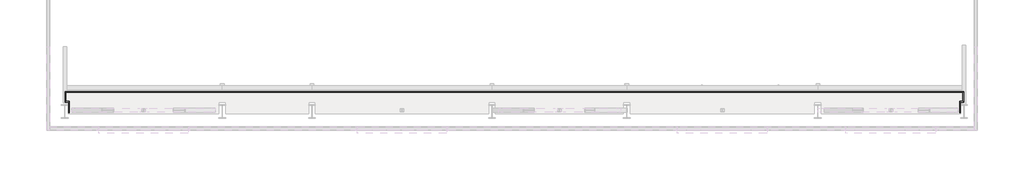
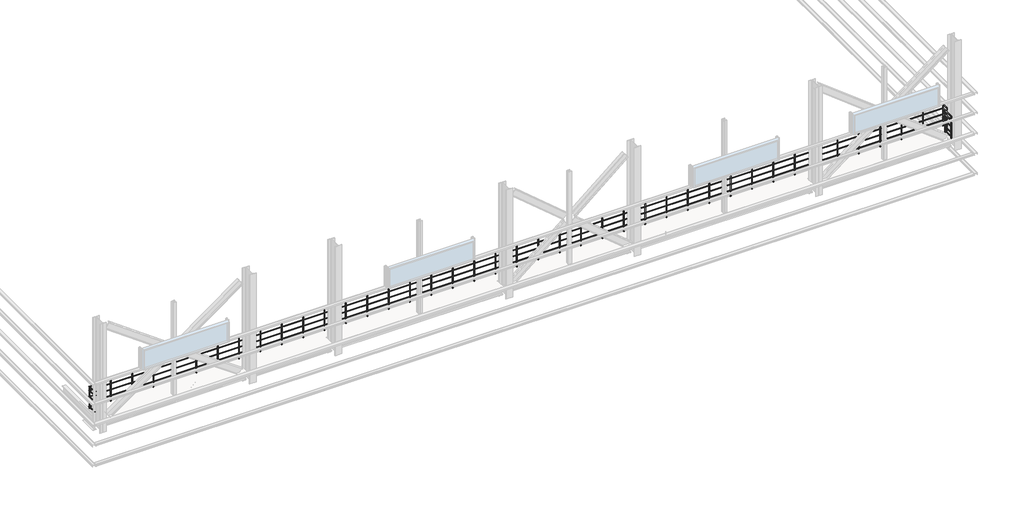
# One storey, part 3 of 4: 1 railing.
"""IFC4 building model written with IfcOpenShell, lengths in millimetres."""

from ifc_helpers import new_model, si_unit, frame, origin, place, context, project, spatial, polyline, circle_curve, ellipse_curve, outline, extrude, element, save
from ifc_brep_helpers import plane_surface, cylinder_surface, advanced_brep

model = new_model("IFC4")

# Units and contexts
model_context = context("Model", 3, world=origin())
ifc_project = project(units=[si_unit("LENGTHUNIT", "METRE", prefix="MILLI")], contexts=[model_context])

# Site, building, storey
site = spatial("IfcSite", under=ifc_project)
building = spatial("IfcBuilding", under=site)
storey = spatial("IfcBuildingStorey", under=building, Name="T.O.CRANE GIR.", Elevation=12299.9720055)

# Railing
placement = place(None, origin())
element("IfcRailing", 1, ObjectType="RA101_1100mm", at=placement, inside=storey, context=model_context, shape_type="SolidModel", body=[
    advanced_brep(
    [(195.0, 20879.5208589, 13466.9720055), (165.0, 20879.5208589, 13466.9720055), (195.0, 21394.5208589, 13466.9720055), (165.0, 21364.5208589, 13466.9720055), (45.0, 21394.5208589, 13466.9720055), (15.0, 21364.5208589, 13466.9720055), (45.0, 21804.5208589, 13466.9720055), (15.0, 21834.5208589, 13466.9720055), (39955.0, 21804.5208589, 13466.9720055), (39985.0, 21834.5208589, 13466.9720055), (39955.0, 21394.5208589, 13466.9720055), (39985.0, 21364.5208589, 13466.9720055), (39805.0, 21394.5208589, 13466.9720055), (39835.0, 21364.5208589, 13466.9720055), (39805.0, 20879.5208589, 13466.9720055), (39835.0, 20879.5208589, 13466.9720055)],
    [
        (0, 1, circle_curve(frame((180.0, 20879.5208589, 13466.9720055), z_axis=(0.0, -1.0, 0.0), x_axis=(-1.0, 0.0, 0.0)), 15.0)),
        (1, 0, circle_curve(frame((180.0, 20879.5208589, 13466.9720055), z_axis=(0.0, -1.0, 0.0), x_axis=(-1.0, 0.0, 0.0)), 15.0)),
        (0, 2),
        (2, 3, ellipse_curve(frame((180.0, 21379.5208589, 13466.9720055), z_axis=(0.7071067811865434, -0.7071067811865516, 0.0), x_axis=(-0.7071067811865516, -0.7071067811865435, 0.0)), 21.2132034, 15.0)),
        (3, 1),
        (3, 2, ellipse_curve(frame((180.0, 21379.5208589, 13466.9720055), z_axis=(0.7071067811865434, -0.7071067811865516, 0.0), x_axis=(-0.7071067811865516, -0.7071067811865435, 0.0)), 21.2132034, 15.0)),
        (2, 4),
        (4, 5, ellipse_curve(frame((30.0, 21379.5208589, 13466.9720055), z_axis=(0.7071067811865434, -0.7071067811865517, 0.0), x_axis=(0.7071067811865517, 0.7071067811865432, 0.0)), 21.2132034, 15.0)),
        (5, 3),
        (5, 4, ellipse_curve(frame((30.0, 21379.5208589, 13466.9720055), z_axis=(0.7071067811865434, -0.7071067811865517, 0.0), x_axis=(0.7071067811865517, 0.7071067811865432, 0.0)), 21.2132034, 15.0)),
        (4, 6),
        (6, 7, ellipse_curve(frame((30.0, 21819.5208589, 13466.9720055), z_axis=(-0.7071067811865507, -0.7071067811865444, 0.0), x_axis=(0.7071067811865442, -0.7071067811865507, 0.0)), 21.2132034, 15.0)),
        (7, 5),
        (7, 6, ellipse_curve(frame((30.0, 21819.5208589, 13466.9720055), z_axis=(-0.7071067811865507, -0.7071067811865444, 0.0), x_axis=(0.7071067811865442, -0.7071067811865507, 0.0)), 21.2132034, 15.0)),
        (6, 8),
        (8, 9, ellipse_curve(frame((39970.0, 21819.5208589, 13466.9720055), z_axis=(-0.7071067811865438, 0.7071067811865512, 0.0), x_axis=(-0.7071067811865512, -0.7071067811865438, 0.0)), 21.2132034, 15.0)),
        (9, 7),
        (9, 8, ellipse_curve(frame((39970.0, 21819.5208589, 13466.9720055), z_axis=(-0.7071067811865438, 0.7071067811865512, 0.0), x_axis=(-0.7071067811865512, -0.7071067811865438, 0.0)), 21.2132034, 15.0)),
        (8, 10),
        (10, 11, ellipse_curve(frame((39970.0, 21379.5208589, 13466.9720055), z_axis=(0.7071067811865525, 0.7071067811865426, 0.0), x_axis=(-0.7071067811865426, 0.7071067811865525, 0.0)), 21.2132034, 15.0)),
        (11, 9),
        (11, 10, ellipse_curve(frame((39970.0, 21379.5208589, 13466.9720055), z_axis=(0.7071067811865525, 0.7071067811865426, 0.0), x_axis=(-0.7071067811865426, 0.7071067811865525, 0.0)), 21.2132034, 15.0)),
        (10, 12),
        (12, 13, ellipse_curve(frame((39820.0, 21379.5208589, 13466.9720055), z_axis=(0.7071067811865525, 0.7071067811865425, 0.0), x_axis=(0.7071067811865426, -0.7071067811865523, 0.0)), 21.2132034, 15.0)),
        (13, 11),
        (13, 12, ellipse_curve(frame((39820.0, 21379.5208589, 13466.9720055), z_axis=(0.7071067811865525, 0.7071067811865425, 0.0), x_axis=(0.7071067811865426, -0.7071067811865523, 0.0)), 21.2132034, 15.0)),
        (14, 15, circle_curve(frame((39820.0, 20879.5208589, 13466.9720055), z_axis=(0.0, -1.0, 0.0), x_axis=(1.0, 0.0, 0.0)), 15.0)),
        (15, 14, circle_curve(frame((39820.0, 20879.5208589, 13466.9720055), z_axis=(0.0, -1.0, 0.0), x_axis=(1.0, 0.0, 0.0)), 15.0)),
        (12, 14),
        (15, 13),
    ],
    [
        plane_surface(frame((180.0, 20879.5208589, 13481.9720055), z_axis=(0.0, -1.0, 0.0), x_axis=(0.0, 0.0, 1.0))),
        cylinder_surface(frame((180.0, 20879.5208589, 13466.9720055), z_axis=(0.0, -1.0, 0.0), x_axis=(-1.0, 0.0, 0.0)), 15.0),
        cylinder_surface(frame((180.0, 21379.5208589, 13466.9720055), z_axis=(1.0, 0.0, 0.0), x_axis=(0.0, -1.0, 0.0)), 15.0),
        cylinder_surface(frame((30.0, 21379.5208589, 13466.9720055), z_axis=(0.0, -1.0, 0.0), x_axis=(-1.0, 0.0, 0.0)), 15.0),
        cylinder_surface(frame((30.0, 21819.5208589, 13466.9720055), z_axis=(-1.0, 0.0, 0.0), x_axis=(0.0, 1.0, 0.0)), 15.0),
        cylinder_surface(frame((39970.0, 21819.5208589, 13466.9720055), z_axis=(0.0, 1.0, 0.0), x_axis=(1.0, 0.0, 0.0)), 15.0),
        cylinder_surface(frame((39970.0, 21379.5208589, 13466.9720055), z_axis=(1.0, 0.0, 0.0), x_axis=(0.0, -1.0, 0.0)), 15.0),
        plane_surface(frame((39820.0, 20879.5208589, 13481.9720055), z_axis=(0.0, -1.0, 0.0), x_axis=(0.0, 0.0, -1.0))),
        cylinder_surface(frame((39820.0, 21379.5208589, 13466.9720055), z_axis=(0.0, 1.0, 0.0), x_axis=(1.0, 0.0, 0.0)), 15.0),
    ],
    [
        (0, [[1, 2]]),
        (1, [[-1, 3, 4, 5]]),
        (1, [[-2, -5, 6, -3]]),
        (2, [[-4, 7, 8, 9]]),
        (2, [[-6, -9, 10, -7]]),
        (3, [[-8, 11, 12, 13]]),
        (3, [[-10, -13, 14, -11]]),
        (4, [[-12, 15, 16, 17]]),
        (4, [[-14, -17, 18, -15]]),
        (5, [[-16, 19, 20, 21]]),
        (5, [[-18, -21, 22, -19]]),
        (6, [[-20, 23, 24, 25]]),
        (6, [[-22, -25, 26, -23]]),
        (7, [[27, 28]]),
        (8, [[-24, 29, -28, 30]]),
        (8, [[-26, -30, -27, -29]]),
    ],
),
    advanced_brep(
    [(45.0, 21394.5208589, 13266.9720055), (15.0, 21364.5208589, 13266.9720055), (15.0, 21834.5208589, 13266.9720055), (45.0, 21804.5208589, 13266.9720055), (39985.0, 21834.5208589, 13266.9720055), (39955.0, 21804.5208589, 13266.9720055), (39985.0, 21364.5208589, 13266.9720055), (39955.0, 21394.5208589, 13266.9720055), (39835.0, 21364.5208589, 13266.9720055), (39805.0, 21394.5208589, 13266.9720055), (39805.0, 20879.5208589, 13266.9720055), (39835.0, 20879.5208589, 13266.9720055), (195.0, 20879.5208589, 13266.9720055), (165.0, 20879.5208589, 13266.9720055), (165.0, 21364.5208589, 13266.9720055), (195.0, 21394.5208589, 13266.9720055)],
    [
        (0, 1, ellipse_curve(frame((30.0, 21379.5208589, 13266.9720055), z_axis=(-0.7071067811865434, 0.7071067811865517, 0.0), x_axis=(-0.7071067811865518, -0.7071067811865434, 0.0)), 21.2132034, 15.0)),
        (1, 2),
        (2, 3, ellipse_curve(frame((30.0, 21819.5208589, 13266.9720055), z_axis=(-0.7071067811865507, -0.7071067811865444, 0.0), x_axis=(0.7071067811865442, -0.7071067811865507, 0.0)), 21.2132034, 15.0)),
        (3, 0),
        (1, 0, ellipse_curve(frame((30.0, 21379.5208589, 13266.9720055), z_axis=(-0.7071067811865434, 0.7071067811865517, 0.0), x_axis=(-0.7071067811865518, -0.7071067811865434, 0.0)), 21.2132034, 15.0)),
        (3, 2, ellipse_curve(frame((30.0, 21819.5208589, 13266.9720055), z_axis=(-0.7071067811865507, -0.7071067811865444, 0.0), x_axis=(0.7071067811865442, -0.7071067811865507, 0.0)), 21.2132034, 15.0)),
        (2, 4),
        (4, 5, ellipse_curve(frame((39970.0, 21819.5208589, 13266.9720055), z_axis=(-0.7071067811865438, 0.7071067811865512, 0.0), x_axis=(-0.7071067811865512, -0.7071067811865438, 0.0)), 21.2132034, 15.0)),
        (5, 3),
        (5, 4, ellipse_curve(frame((39970.0, 21819.5208589, 13266.9720055), z_axis=(-0.7071067811865438, 0.7071067811865512, 0.0), x_axis=(-0.7071067811865512, -0.7071067811865438, 0.0)), 21.2132034, 15.0)),
        (4, 6),
        (6, 7, ellipse_curve(frame((39970.0, 21379.5208589, 13266.9720055), z_axis=(0.7071067811865525, 0.7071067811865426, 0.0), x_axis=(-0.7071067811865426, 0.7071067811865525, 0.0)), 21.2132034, 15.0)),
        (7, 5),
        (7, 6, ellipse_curve(frame((39970.0, 21379.5208589, 13266.9720055), z_axis=(0.7071067811865525, 0.7071067811865426, 0.0), x_axis=(-0.7071067811865426, 0.7071067811865525, 0.0)), 21.2132034, 15.0)),
        (6, 8),
        (8, 9, ellipse_curve(frame((39820.0, 21379.5208589, 13266.9720055), z_axis=(0.7071067811865525, 0.7071067811865425, 0.0), x_axis=(0.7071067811865426, -0.7071067811865523, 0.0)), 21.2132034, 15.0)),
        (9, 7),
        (9, 8, ellipse_curve(frame((39820.0, 21379.5208589, 13266.9720055), z_axis=(0.7071067811865525, 0.7071067811865425, 0.0), x_axis=(0.7071067811865426, -0.7071067811865523, 0.0)), 21.2132034, 15.0)),
        (10, 11, circle_curve(frame((39820.0, 20879.5208589, 13266.9720055), z_axis=(0.0, -1.0, 0.0), x_axis=(1.0, 0.0, 0.0)), 15.0)),
        (11, 10, circle_curve(frame((39820.0, 20879.5208589, 13266.9720055), z_axis=(0.0, -1.0, 0.0), x_axis=(1.0, 0.0, 0.0)), 15.0)),
        (8, 11),
        (10, 9),
        (12, 13, circle_curve(frame((180.0, 20879.5208589, 13266.9720055), z_axis=(0.0, -1.0, 0.0), x_axis=(-1.0, 0.0, 0.0)), 15.0)),
        (13, 12, circle_curve(frame((180.0, 20879.5208589, 13266.9720055), z_axis=(0.0, -1.0, 0.0), x_axis=(-1.0, 0.0, 0.0)), 15.0)),
        (13, 14),
        (14, 15, ellipse_curve(frame((180.0, 21379.5208589, 13266.9720055), z_axis=(0.7071067811865434, -0.7071067811865516, 0.0), x_axis=(-0.7071067811865516, -0.7071067811865435, 0.0)), 21.2132034, 15.0)),
        (15, 12),
        (15, 14, ellipse_curve(frame((180.0, 21379.5208589, 13266.9720055), z_axis=(0.7071067811865434, -0.7071067811865516, 0.0), x_axis=(-0.7071067811865516, -0.7071067811865435, 0.0)), 21.2132034, 15.0)),
        (14, 1),
        (0, 15),
    ],
    [
        cylinder_surface(frame((30.0, 21379.5208589, 13266.9720055), z_axis=(0.0, -1.0, 0.0), x_axis=(-1.0, 0.0, 0.0)), 15.0),
        cylinder_surface(frame((30.0, 21819.5208589, 13266.9720055), z_axis=(-1.0, 0.0, 0.0), x_axis=(0.0, 1.0, 0.0)), 15.0),
        cylinder_surface(frame((39970.0, 21819.5208589, 13266.9720055), z_axis=(0.0, 1.0, 0.0), x_axis=(1.0, 0.0, 0.0)), 15.0),
        cylinder_surface(frame((39970.0, 21379.5208589, 13266.9720055), z_axis=(1.0, 0.0, 0.0), x_axis=(0.0, -1.0, 0.0)), 15.0),
        plane_surface(frame((39820.0, 20879.5208589, 13281.9720055), z_axis=(0.0, -1.0, 0.0), x_axis=(0.0, 0.0, -1.0))),
        cylinder_surface(frame((39820.0, 21379.5208589, 13266.9720055), z_axis=(0.0, 1.0, 0.0), x_axis=(1.0, 0.0, 0.0)), 15.0),
        plane_surface(frame((180.0, 20879.5208589, 13281.9720055), z_axis=(0.0, -1.0, 0.0), x_axis=(0.0, 0.0, 1.0))),
        cylinder_surface(frame((180.0, 20879.5208589, 13266.9720055), z_axis=(0.0, -1.0, 0.0), x_axis=(-1.0, 0.0, 0.0)), 15.0),
        cylinder_surface(frame((180.0, 21379.5208589, 13266.9720055), z_axis=(1.0, 0.0, 0.0), x_axis=(0.0, -1.0, 0.0)), 15.0),
    ],
    [
        (0, [[1, 2, 3, 4]]),
        (0, [[5, -4, 6, -2]]),
        (1, [[-3, 7, 8, 9]]),
        (1, [[-6, -9, 10, -7]]),
        (2, [[-8, 11, 12, 13]]),
        (2, [[-10, -13, 14, -11]]),
        (3, [[-12, 15, 16, 17]]),
        (3, [[-14, -17, 18, -15]]),
        (4, [[19, 20]]),
        (5, [[-16, 21, -19, 22]]),
        (5, [[-18, -22, -20, -21]]),
        (6, [[23, 24]]),
        (7, [[-24, 25, 26, 27]]),
        (7, [[-23, -27, 28, -25]]),
        (8, [[-26, 29, -1, 30]]),
        (8, [[-28, -30, -5, -29]]),
    ],
),
    advanced_brep(
    [(45.0, 21394.5208589, 12966.9720055), (15.0, 21364.5208589, 12966.9720055), (15.0, 21834.5208589, 12966.9720055), (45.0, 21804.5208589, 12966.9720055), (39985.0, 21834.5208589, 12966.9720055), (39955.0, 21804.5208589, 12966.9720055), (39985.0, 21364.5208589, 12966.9720055), (39955.0, 21394.5208589, 12966.9720055), (39835.0, 21364.5208589, 12966.9720055), (39805.0, 21394.5208589, 12966.9720055), (39805.0, 20879.5208589, 12966.9720055), (39835.0, 20879.5208589, 12966.9720055), (195.0, 20879.5208589, 12966.9720055), (165.0, 20879.5208589, 12966.9720055), (165.0, 21364.5208589, 12966.9720055), (195.0, 21394.5208589, 12966.9720055)],
    [
        (0, 1, ellipse_curve(frame((30.0, 21379.5208589, 12966.9720055), z_axis=(-0.7071067811865434, 0.7071067811865517, 0.0), x_axis=(-0.7071067811865518, -0.7071067811865434, 0.0)), 21.2132034, 15.0)),
        (1, 2),
        (2, 3, ellipse_curve(frame((30.0, 21819.5208589, 12966.9720055), z_axis=(-0.7071067811865507, -0.7071067811865444, 0.0), x_axis=(0.7071067811865442, -0.7071067811865507, 0.0)), 21.2132034, 15.0)),
        (3, 0),
        (1, 0, ellipse_curve(frame((30.0, 21379.5208589, 12966.9720055), z_axis=(-0.7071067811865434, 0.7071067811865517, 0.0), x_axis=(-0.7071067811865518, -0.7071067811865434, 0.0)), 21.2132034, 15.0)),
        (3, 2, ellipse_curve(frame((30.0, 21819.5208589, 12966.9720055), z_axis=(-0.7071067811865507, -0.7071067811865444, 0.0), x_axis=(0.7071067811865442, -0.7071067811865507, 0.0)), 21.2132034, 15.0)),
        (2, 4),
        (4, 5, ellipse_curve(frame((39970.0, 21819.5208589, 12966.9720055), z_axis=(-0.7071067811865438, 0.7071067811865512, 0.0), x_axis=(-0.7071067811865512, -0.7071067811865438, 0.0)), 21.2132034, 15.0)),
        (5, 3),
        (5, 4, ellipse_curve(frame((39970.0, 21819.5208589, 12966.9720055), z_axis=(-0.7071067811865438, 0.7071067811865512, 0.0), x_axis=(-0.7071067811865512, -0.7071067811865438, 0.0)), 21.2132034, 15.0)),
        (4, 6),
        (6, 7, ellipse_curve(frame((39970.0, 21379.5208589, 12966.9720055), z_axis=(0.7071067811865525, 0.7071067811865426, 0.0), x_axis=(-0.7071067811865426, 0.7071067811865525, 0.0)), 21.2132034, 15.0)),
        (7, 5),
        (7, 6, ellipse_curve(frame((39970.0, 21379.5208589, 12966.9720055), z_axis=(0.7071067811865525, 0.7071067811865426, 0.0), x_axis=(-0.7071067811865426, 0.7071067811865525, 0.0)), 21.2132034, 15.0)),
        (6, 8),
        (8, 9, ellipse_curve(frame((39820.0, 21379.5208589, 12966.9720055), z_axis=(0.7071067811865525, 0.7071067811865425, 0.0), x_axis=(0.7071067811865426, -0.7071067811865523, 0.0)), 21.2132034, 15.0)),
        (9, 7),
        (9, 8, ellipse_curve(frame((39820.0, 21379.5208589, 12966.9720055), z_axis=(0.7071067811865525, 0.7071067811865425, 0.0), x_axis=(0.7071067811865426, -0.7071067811865523, 0.0)), 21.2132034, 15.0)),
        (10, 11, circle_curve(frame((39820.0, 20879.5208589, 12966.9720055), z_axis=(0.0, -1.0, 0.0), x_axis=(1.0, 0.0, 0.0)), 15.0)),
        (11, 10, circle_curve(frame((39820.0, 20879.5208589, 12966.9720055), z_axis=(0.0, -1.0, 0.0), x_axis=(1.0, 0.0, 0.0)), 15.0)),
        (8, 11),
        (10, 9),
        (12, 13, circle_curve(frame((180.0, 20879.5208589, 12966.9720055), z_axis=(0.0, -1.0, 0.0), x_axis=(-1.0, 0.0, 0.0)), 15.0)),
        (13, 12, circle_curve(frame((180.0, 20879.5208589, 12966.9720055), z_axis=(0.0, -1.0, 0.0), x_axis=(-1.0, 0.0, 0.0)), 15.0)),
        (13, 14),
        (14, 15, ellipse_curve(frame((180.0, 21379.5208589, 12966.9720055), z_axis=(0.7071067811865434, -0.7071067811865516, 0.0), x_axis=(-0.7071067811865516, -0.7071067811865435, 0.0)), 21.2132034, 15.0)),
        (15, 12),
        (15, 14, ellipse_curve(frame((180.0, 21379.5208589, 12966.9720055), z_axis=(0.7071067811865434, -0.7071067811865516, 0.0), x_axis=(-0.7071067811865516, -0.7071067811865435, 0.0)), 21.2132034, 15.0)),
        (14, 1),
        (0, 15),
    ],
    [
        cylinder_surface(frame((30.0, 21379.5208589, 12966.9720055), z_axis=(0.0, -1.0, 0.0), x_axis=(-1.0, 0.0, 0.0)), 15.0),
        cylinder_surface(frame((30.0, 21819.5208589, 12966.9720055), z_axis=(-1.0, 0.0, 0.0), x_axis=(0.0, 1.0, 0.0)), 15.0),
        cylinder_surface(frame((39970.0, 21819.5208589, 12966.9720055), z_axis=(0.0, 1.0, 0.0), x_axis=(1.0, 0.0, 0.0)), 15.0),
        cylinder_surface(frame((39970.0, 21379.5208589, 12966.9720055), z_axis=(1.0, 0.0, 0.0), x_axis=(0.0, -1.0, 0.0)), 15.0),
        plane_surface(frame((39820.0, 20879.5208589, 12981.9720055), z_axis=(0.0, -1.0, 0.0), x_axis=(0.0, 0.0, -1.0))),
        cylinder_surface(frame((39820.0, 21379.5208589, 12966.9720055), z_axis=(0.0, 1.0, 0.0), x_axis=(1.0, 0.0, 0.0)), 15.0),
        plane_surface(frame((180.0, 20879.5208589, 12981.9720055), z_axis=(0.0, -1.0, 0.0), x_axis=(0.0, 0.0, 1.0))),
        cylinder_surface(frame((180.0, 20879.5208589, 12966.9720055), z_axis=(0.0, -1.0, 0.0), x_axis=(-1.0, 0.0, 0.0)), 15.0),
        cylinder_surface(frame((180.0, 21379.5208589, 12966.9720055), z_axis=(1.0, 0.0, 0.0), x_axis=(0.0, -1.0, 0.0)), 15.0),
    ],
    [
        (0, [[1, 2, 3, 4]]),
        (0, [[5, -4, 6, -2]]),
        (1, [[-3, 7, 8, 9]]),
        (1, [[-6, -9, 10, -7]]),
        (2, [[-8, 11, 12, 13]]),
        (2, [[-10, -13, 14, -11]]),
        (3, [[-12, 15, 16, 17]]),
        (3, [[-14, -17, 18, -15]]),
        (4, [[19, 20]]),
        (5, [[-16, 21, -19, 22]]),
        (5, [[-18, -22, -20, -21]]),
        (6, [[23, 24]]),
        (7, [[-24, 25, 26, 27]]),
        (7, [[-23, -27, 28, -25]]),
        (8, [[-26, 29, -1, 30]]),
        (8, [[-28, -30, -5, -29]]),
    ],
),
    advanced_brep(
    [(195.0, 20879.5208589, 12666.9720055), (165.0, 20879.5208589, 12666.9720055), (195.0, 21394.5208589, 12666.9720055), (165.0, 21364.5208589, 12666.9720055), (45.0, 21394.5208589, 12666.9720055), (15.0, 21364.5208589, 12666.9720055), (45.0, 21804.5208589, 12666.9720055), (15.0, 21834.5208589, 12666.9720055), (39955.0, 21804.5208589, 12666.9720055), (39985.0, 21834.5208589, 12666.9720055), (39955.0, 21394.5208589, 12666.9720055), (39985.0, 21364.5208589, 12666.9720055), (39805.0, 21394.5208589, 12666.9720055), (39835.0, 21364.5208589, 12666.9720055), (39805.0, 20879.5208589, 12666.9720055), (39835.0, 20879.5208589, 12666.9720055)],
    [
        (0, 1, circle_curve(frame((180.0, 20879.5208589, 12666.9720055), z_axis=(0.0, -1.0, 0.0), x_axis=(-1.0, 0.0, 0.0)), 15.0)),
        (1, 0, circle_curve(frame((180.0, 20879.5208589, 12666.9720055), z_axis=(0.0, -1.0, 0.0), x_axis=(-1.0, 0.0, 0.0)), 15.0)),
        (0, 2),
        (2, 3, ellipse_curve(frame((180.0, 21379.5208589, 12666.9720055), z_axis=(0.7071067811865434, -0.7071067811865516, 0.0), x_axis=(-0.7071067811865516, -0.7071067811865435, 0.0)), 21.2132034, 15.0)),
        (3, 1),
        (3, 2, ellipse_curve(frame((180.0, 21379.5208589, 12666.9720055), z_axis=(0.7071067811865434, -0.7071067811865516, 0.0), x_axis=(-0.7071067811865516, -0.7071067811865435, 0.0)), 21.2132034, 15.0)),
        (2, 4),
        (4, 5, ellipse_curve(frame((30.0, 21379.5208589, 12666.9720055), z_axis=(0.7071067811865434, -0.7071067811865517, 0.0), x_axis=(0.7071067811865517, 0.7071067811865432, 0.0)), 21.2132034, 15.0)),
        (5, 3),
        (5, 4, ellipse_curve(frame((30.0, 21379.5208589, 12666.9720055), z_axis=(0.7071067811865434, -0.7071067811865517, 0.0), x_axis=(0.7071067811865517, 0.7071067811865432, 0.0)), 21.2132034, 15.0)),
        (4, 6),
        (6, 7, ellipse_curve(frame((30.0, 21819.5208589, 12666.9720055), z_axis=(-0.7071067811865507, -0.7071067811865444, 0.0), x_axis=(0.7071067811865442, -0.7071067811865507, 0.0)), 21.2132034, 15.0)),
        (7, 5),
        (7, 6, ellipse_curve(frame((30.0, 21819.5208589, 12666.9720055), z_axis=(-0.7071067811865507, -0.7071067811865444, 0.0), x_axis=(0.7071067811865442, -0.7071067811865507, 0.0)), 21.2132034, 15.0)),
        (6, 8),
        (8, 9, ellipse_curve(frame((39970.0, 21819.5208589, 12666.9720055), z_axis=(-0.7071067811865438, 0.7071067811865512, 0.0), x_axis=(-0.7071067811865512, -0.7071067811865438, 0.0)), 21.2132034, 15.0)),
        (9, 7),
        (9, 8, ellipse_curve(frame((39970.0, 21819.5208589, 12666.9720055), z_axis=(-0.7071067811865438, 0.7071067811865512, 0.0), x_axis=(-0.7071067811865512, -0.7071067811865438, 0.0)), 21.2132034, 15.0)),
        (8, 10),
        (10, 11, ellipse_curve(frame((39970.0, 21379.5208589, 12666.9720055), z_axis=(0.7071067811865525, 0.7071067811865426, 0.0), x_axis=(-0.7071067811865426, 0.7071067811865525, 0.0)), 21.2132034, 15.0)),
        (11, 9),
        (11, 10, ellipse_curve(frame((39970.0, 21379.5208589, 12666.9720055), z_axis=(0.7071067811865525, 0.7071067811865426, 0.0), x_axis=(-0.7071067811865426, 0.7071067811865525, 0.0)), 21.2132034, 15.0)),
        (10, 12),
        (12, 13, ellipse_curve(frame((39820.0, 21379.5208589, 12666.9720055), z_axis=(0.7071067811865525, 0.7071067811865425, 0.0), x_axis=(0.7071067811865426, -0.7071067811865523, 0.0)), 21.2132034, 15.0)),
        (13, 11),
        (13, 12, ellipse_curve(frame((39820.0, 21379.5208589, 12666.9720055), z_axis=(0.7071067811865525, 0.7071067811865425, 0.0), x_axis=(0.7071067811865426, -0.7071067811865523, 0.0)), 21.2132034, 15.0)),
        (14, 15, circle_curve(frame((39820.0, 20879.5208589, 12666.9720055), z_axis=(0.0, -1.0, 0.0), x_axis=(1.0, 0.0, 0.0)), 15.0)),
        (15, 14, circle_curve(frame((39820.0, 20879.5208589, 12666.9720055), z_axis=(0.0, -1.0, 0.0), x_axis=(1.0, 0.0, 0.0)), 15.0)),
        (12, 14),
        (15, 13),
    ],
    [
        plane_surface(frame((180.0, 20879.5208589, 12681.9720055), z_axis=(0.0, -1.0, 0.0), x_axis=(0.0, 0.0, 1.0))),
        cylinder_surface(frame((180.0, 20879.5208589, 12666.9720055), z_axis=(0.0, -1.0, 0.0), x_axis=(-1.0, 0.0, 0.0)), 15.0),
        cylinder_surface(frame((180.0, 21379.5208589, 12666.9720055), z_axis=(1.0, 0.0, 0.0), x_axis=(0.0, -1.0, 0.0)), 15.0),
        cylinder_surface(frame((30.0, 21379.5208589, 12666.9720055), z_axis=(0.0, -1.0, 0.0), x_axis=(-1.0, 0.0, 0.0)), 15.0),
        cylinder_surface(frame((30.0, 21819.5208589, 12666.9720055), z_axis=(-1.0, 0.0, 0.0), x_axis=(0.0, 1.0, 0.0)), 15.0),
        cylinder_surface(frame((39970.0, 21819.5208589, 12666.9720055), z_axis=(0.0, 1.0, 0.0), x_axis=(1.0, 0.0, 0.0)), 15.0),
        cylinder_surface(frame((39970.0, 21379.5208589, 12666.9720055), z_axis=(1.0, 0.0, 0.0), x_axis=(0.0, -1.0, 0.0)), 15.0),
        plane_surface(frame((39820.0, 20879.5208589, 12681.9720055), z_axis=(0.0, -1.0, 0.0), x_axis=(0.0, 0.0, -1.0))),
        cylinder_surface(frame((39820.0, 21379.5208589, 12666.9720055), z_axis=(0.0, 1.0, 0.0), x_axis=(1.0, 0.0, 0.0)), 15.0),
    ],
    [
        (0, [[1, 2]]),
        (1, [[-1, 3, 4, 5]]),
        (1, [[-2, -5, 6, -3]]),
        (2, [[-4, 7, 8, 9]]),
        (2, [[-6, -9, 10, -7]]),
        (3, [[-8, 11, 12, 13]]),
        (3, [[-10, -13, 14, -11]]),
        (4, [[-12, 15, 16, 17]]),
        (4, [[-14, -17, 18, -15]]),
        (5, [[-16, 19, 20, 21]]),
        (5, [[-18, -21, 22, -19]]),
        (6, [[-20, 23, 24, 25]]),
        (6, [[-22, -25, 26, -23]]),
        (7, [[27, 28]]),
        (8, [[-24, 29, -28, 30]]),
        (8, [[-26, -30, -27, -29]]),
    ],
),
    advanced_brep(
    [(195.0, 20879.5208589, 12466.9720055), (165.0, 20879.5208589, 12466.9720055), (195.0, 21394.5208589, 12466.9720055), (165.0, 21364.5208589, 12466.9720055), (45.0, 21394.5208589, 12466.9720055), (15.0, 21364.5208589, 12466.9720055), (45.0, 21804.5208589, 12466.9720055), (15.0, 21834.5208589, 12466.9720055), (39955.0, 21804.5208589, 12466.9720055), (39985.0, 21834.5208589, 12466.9720055), (39955.0, 21394.5208589, 12466.9720055), (39985.0, 21364.5208589, 12466.9720055), (39805.0, 21394.5208589, 12466.9720055), (39835.0, 21364.5208589, 12466.9720055), (39805.0, 20879.5208589, 12466.9720055), (39835.0, 20879.5208589, 12466.9720055)],
    [
        (0, 1, circle_curve(frame((180.0, 20879.5208589, 12466.9720055), z_axis=(0.0, -1.0, 0.0), x_axis=(-1.0, 0.0, 0.0)), 15.0)),
        (1, 0, circle_curve(frame((180.0, 20879.5208589, 12466.9720055), z_axis=(0.0, -1.0, 0.0), x_axis=(-1.0, 0.0, 0.0)), 15.0)),
        (0, 2),
        (2, 3, ellipse_curve(frame((180.0, 21379.5208589, 12466.9720055), z_axis=(0.7071067811865434, -0.7071067811865516, 0.0), x_axis=(-0.7071067811865516, -0.7071067811865435, 0.0)), 21.2132034, 15.0)),
        (3, 1),
        (3, 2, ellipse_curve(frame((180.0, 21379.5208589, 12466.9720055), z_axis=(0.7071067811865434, -0.7071067811865516, 0.0), x_axis=(-0.7071067811865516, -0.7071067811865435, 0.0)), 21.2132034, 15.0)),
        (2, 4),
        (4, 5, ellipse_curve(frame((30.0, 21379.5208589, 12466.9720055), z_axis=(0.7071067811865434, -0.7071067811865517, 0.0), x_axis=(0.7071067811865517, 0.7071067811865432, 0.0)), 21.2132034, 15.0)),
        (5, 3),
        (5, 4, ellipse_curve(frame((30.0, 21379.5208589, 12466.9720055), z_axis=(0.7071067811865434, -0.7071067811865517, 0.0), x_axis=(0.7071067811865517, 0.7071067811865432, 0.0)), 21.2132034, 15.0)),
        (4, 6),
        (6, 7, ellipse_curve(frame((30.0, 21819.5208589, 12466.9720055), z_axis=(-0.7071067811865507, -0.7071067811865444, 0.0), x_axis=(0.7071067811865442, -0.7071067811865507, 0.0)), 21.2132034, 15.0)),
        (7, 5),
        (7, 6, ellipse_curve(frame((30.0, 21819.5208589, 12466.9720055), z_axis=(-0.7071067811865507, -0.7071067811865444, 0.0), x_axis=(0.7071067811865442, -0.7071067811865507, 0.0)), 21.2132034, 15.0)),
        (6, 8),
        (8, 9, ellipse_curve(frame((39970.0, 21819.5208589, 12466.9720055), z_axis=(-0.7071067811865438, 0.7071067811865512, 0.0), x_axis=(-0.7071067811865512, -0.7071067811865438, 0.0)), 21.2132034, 15.0)),
        (9, 7),
        (9, 8, ellipse_curve(frame((39970.0, 21819.5208589, 12466.9720055), z_axis=(-0.7071067811865438, 0.7071067811865512, 0.0), x_axis=(-0.7071067811865512, -0.7071067811865438, 0.0)), 21.2132034, 15.0)),
        (8, 10),
        (10, 11, ellipse_curve(frame((39970.0, 21379.5208589, 12466.9720055), z_axis=(0.7071067811865525, 0.7071067811865426, 0.0), x_axis=(-0.7071067811865426, 0.7071067811865525, 0.0)), 21.2132034, 15.0)),
        (11, 9),
        (11, 10, ellipse_curve(frame((39970.0, 21379.5208589, 12466.9720055), z_axis=(0.7071067811865525, 0.7071067811865426, 0.0), x_axis=(-0.7071067811865426, 0.7071067811865525, 0.0)), 21.2132034, 15.0)),
        (10, 12),
        (12, 13, ellipse_curve(frame((39820.0, 21379.5208589, 12466.9720055), z_axis=(0.7071067811865525, 0.7071067811865425, 0.0), x_axis=(0.7071067811865426, -0.7071067811865523, 0.0)), 21.2132034, 15.0)),
        (13, 11),
        (13, 12, ellipse_curve(frame((39820.0, 21379.5208589, 12466.9720055), z_axis=(0.7071067811865525, 0.7071067811865425, 0.0), x_axis=(0.7071067811865426, -0.7071067811865523, 0.0)), 21.2132034, 15.0)),
        (14, 15, circle_curve(frame((39820.0, 20879.5208589, 12466.9720055), z_axis=(0.0, -1.0, 0.0), x_axis=(1.0, 0.0, 0.0)), 15.0)),
        (15, 14, circle_curve(frame((39820.0, 20879.5208589, 12466.9720055), z_axis=(0.0, -1.0, 0.0), x_axis=(1.0, 0.0, 0.0)), 15.0)),
        (12, 14),
        (15, 13),
    ],
    [
        plane_surface(frame((180.0, 20879.5208589, 12481.9720055), z_axis=(0.0, -1.0, 0.0), x_axis=(0.0, 0.0, 1.0))),
        cylinder_surface(frame((180.0, 20879.5208589, 12466.9720055), z_axis=(0.0, -1.0, 0.0), x_axis=(-1.0, 0.0, 0.0)), 15.0),
        cylinder_surface(frame((180.0, 21379.5208589, 12466.9720055), z_axis=(1.0, 0.0, 0.0), x_axis=(0.0, -1.0, 0.0)), 15.0),
        cylinder_surface(frame((30.0, 21379.5208589, 12466.9720055), z_axis=(0.0, -1.0, 0.0), x_axis=(-1.0, 0.0, 0.0)), 15.0),
        cylinder_surface(frame((30.0, 21819.5208589, 12466.9720055), z_axis=(-1.0, 0.0, 0.0), x_axis=(0.0, 1.0, 0.0)), 15.0),
        cylinder_surface(frame((39970.0, 21819.5208589, 12466.9720055), z_axis=(0.0, 1.0, 0.0), x_axis=(1.0, 0.0, 0.0)), 15.0),
        cylinder_surface(frame((39970.0, 21379.5208589, 12466.9720055), z_axis=(1.0, 0.0, 0.0), x_axis=(0.0, -1.0, 0.0)), 15.0),
        plane_surface(frame((39820.0, 20879.5208589, 12481.9720055), z_axis=(0.0, -1.0, 0.0), x_axis=(0.0, 0.0, -1.0))),
        cylinder_surface(frame((39820.0, 21379.5208589, 12466.9720055), z_axis=(0.0, 1.0, 0.0), x_axis=(1.0, 0.0, 0.0)), 15.0),
    ],
    [
        (0, [[1, 2]]),
        (1, [[-1, 3, 4, 5]]),
        (1, [[-2, -5, 6, -3]]),
        (2, [[-4, 7, 8, 9]]),
        (2, [[-6, -9, 10, -7]]),
        (3, [[-8, 11, 12, 13]]),
        (3, [[-10, -13, 14, -11]]),
        (4, [[-12, 15, 16, 17]]),
        (4, [[-14, -17, 18, -15]]),
        (5, [[-16, 19, 20, 21]]),
        (5, [[-18, -21, 22, -19]]),
        (6, [[-20, 23, 24, 25]]),
        (6, [[-22, -25, 26, -23]]),
        (7, [[27, 28]]),
        (8, [[-24, 29, -28, 30]]),
        (8, [[-26, -30, -27, -29]]),
    ],
),
    extrude(outline(polyline([(39017.5, 21832.0208589), (39042.5, 21832.0208589), (39042.5, 21807.0208589), (39017.5, 21807.0208589), (39017.5, 21832.0208589)])), frame((0.0, 0.0, 12381.9720055), z_axis=(0.0, 0.0, 1.0), x_axis=(1.0, 0.0, 0.0)), (0.0, 0.0, 1.0), 1070.0),
    extrude(outline(polyline([(38017.5, 21832.0208589), (38042.5, 21832.0208589), (38042.5, 21807.0208589), (38017.5, 21807.0208589), (38017.5, 21832.0208589)])), frame((0.0, 0.0, 12381.9720055), z_axis=(0.0, 0.0, 1.0), x_axis=(1.0, 0.0, 0.0)), (0.0, 0.0, 1.0), 1070.0),
    extrude(outline(polyline([(37017.5, 21832.0208589), (37042.5, 21832.0208589), (37042.5, 21807.0208589), (37017.5, 21807.0208589), (37017.5, 21832.0208589)])), frame((0.0, 0.0, 12381.9720055), z_axis=(0.0, 0.0, 1.0), x_axis=(1.0, 0.0, 0.0)), (0.0, 0.0, 1.0), 1070.0),
    extrude(outline(polyline([(36017.5, 21832.0208589), (36042.5, 21832.0208589), (36042.5, 21807.0208589), (36017.5, 21807.0208589), (36017.5, 21832.0208589)])), frame((0.0, 0.0, 12381.9720055), z_axis=(0.0, 0.0, 1.0), x_axis=(1.0, 0.0, 0.0)), (0.0, 0.0, 1.0), 1070.0),
    extrude(outline(polyline([(35017.5, 21832.0208589), (35042.5, 21832.0208589), (35042.5, 21807.0208589), (35017.5, 21807.0208589), (35017.5, 21832.0208589)])), frame((0.0, 0.0, 12381.9720055), z_axis=(0.0, 0.0, 1.0), x_axis=(1.0, 0.0, 0.0)), (0.0, 0.0, 1.0), 1070.0),
    extrude(outline(polyline([(34017.5, 21832.0208589), (34042.5, 21832.0208589), (34042.5, 21807.0208589), (34017.5, 21807.0208589), (34017.5, 21832.0208589)])), frame((0.0, 0.0, 12381.9720055), z_axis=(0.0, 0.0, 1.0), x_axis=(1.0, 0.0, 0.0)), (0.0, 0.0, 1.0), 1070.0),
    extrude(outline(polyline([(33017.5, 21832.0208589), (33042.5, 21832.0208589), (33042.5, 21807.0208589), (33017.5, 21807.0208589), (33017.5, 21832.0208589)])), frame((0.0, 0.0, 12381.9720055), z_axis=(0.0, 0.0, 1.0), x_axis=(1.0, 0.0, 0.0)), (0.0, 0.0, 1.0), 1070.0),
    extrude(outline(polyline([(32017.5, 21832.0208589), (32042.5, 21832.0208589), (32042.5, 21807.0208589), (32017.5, 21807.0208589), (32017.5, 21832.0208589)])), frame((0.0, 0.0, 12381.9720055), z_axis=(0.0, 0.0, 1.0), x_axis=(1.0, 0.0, 0.0)), (0.0, 0.0, 1.0), 1070.0),
    extrude(outline(polyline([(31017.5, 21832.0208589), (31042.5, 21832.0208589), (31042.5, 21807.0208589), (31017.5, 21807.0208589), (31017.5, 21832.0208589)])), frame((0.0, 0.0, 12381.9720055), z_axis=(0.0, 0.0, 1.0), x_axis=(1.0, 0.0, 0.0)), (0.0, 0.0, 1.0), 1070.0),
    extrude(outline(polyline([(30017.5, 21832.0208589), (30042.5, 21832.0208589), (30042.5, 21807.0208589), (30017.5, 21807.0208589), (30017.5, 21832.0208589)])), frame((0.0, 0.0, 12381.9720055), z_axis=(0.0, 0.0, 1.0), x_axis=(1.0, 0.0, 0.0)), (0.0, 0.0, 1.0), 1070.0),
    extrude(outline(polyline([(29017.5, 21832.0208589), (29042.5, 21832.0208589), (29042.5, 21807.0208589), (29017.5, 21807.0208589), (29017.5, 21832.0208589)])), frame((0.0, 0.0, 12381.9720055), z_axis=(0.0, 0.0, 1.0), x_axis=(1.0, 0.0, 0.0)), (0.0, 0.0, 1.0), 1070.0),
    extrude(outline(polyline([(28017.5, 21832.0208589), (28042.5, 21832.0208589), (28042.5, 21807.0208589), (28017.5, 21807.0208589), (28017.5, 21832.0208589)])), frame((0.0, 0.0, 12381.9720055), z_axis=(0.0, 0.0, 1.0), x_axis=(1.0, 0.0, 0.0)), (0.0, 0.0, 1.0), 1070.0),
    extrude(outline(polyline([(27017.5, 21832.0208589), (27042.5, 21832.0208589), (27042.5, 21807.0208589), (27017.5, 21807.0208589), (27017.5, 21832.0208589)])), frame((0.0, 0.0, 12381.9720055), z_axis=(0.0, 0.0, 1.0), x_axis=(1.0, 0.0, 0.0)), (0.0, 0.0, 1.0), 1070.0),
    extrude(outline(polyline([(26017.5, 21832.0208589), (26042.5, 21832.0208589), (26042.5, 21807.0208589), (26017.5, 21807.0208589), (26017.5, 21832.0208589)])), frame((0.0, 0.0, 12381.9720055), z_axis=(0.0, 0.0, 1.0), x_axis=(1.0, 0.0, 0.0)), (0.0, 0.0, 1.0), 1070.0),
    extrude(outline(polyline([(25017.5, 21832.0208589), (25042.5, 21832.0208589), (25042.5, 21807.0208589), (25017.5, 21807.0208589), (25017.5, 21832.0208589)])), frame((0.0, 0.0, 12381.9720055), z_axis=(0.0, 0.0, 1.0), x_axis=(1.0, 0.0, 0.0)), (0.0, 0.0, 1.0), 1070.0),
    extrude(outline(polyline([(24017.5, 21832.0208589), (24042.5, 21832.0208589), (24042.5, 21807.0208589), (24017.5, 21807.0208589), (24017.5, 21832.0208589)])), frame((0.0, 0.0, 12381.9720055), z_axis=(0.0, 0.0, 1.0), x_axis=(1.0, 0.0, 0.0)), (0.0, 0.0, 1.0), 1070.0),
    extrude(outline(polyline([(23017.5, 21832.0208589), (23042.5, 21832.0208589), (23042.5, 21807.0208589), (23017.5, 21807.0208589), (23017.5, 21832.0208589)])), frame((0.0, 0.0, 12381.9720055), z_axis=(0.0, 0.0, 1.0), x_axis=(1.0, 0.0, 0.0)), (0.0, 0.0, 1.0), 1070.0),
    extrude(outline(polyline([(22017.5, 21832.0208589), (22042.5, 21832.0208589), (22042.5, 21807.0208589), (22017.5, 21807.0208589), (22017.5, 21832.0208589)])), frame((0.0, 0.0, 12381.9720055), z_axis=(0.0, 0.0, 1.0), x_axis=(1.0, 0.0, 0.0)), (0.0, 0.0, 1.0), 1070.0),
    extrude(outline(polyline([(21017.5, 21832.0208589), (21042.5, 21832.0208589), (21042.5, 21807.0208589), (21017.5, 21807.0208589), (21017.5, 21832.0208589)])), frame((0.0, 0.0, 12381.9720055), z_axis=(0.0, 0.0, 1.0), x_axis=(1.0, 0.0, 0.0)), (0.0, 0.0, 1.0), 1070.0),
    extrude(outline(polyline([(20017.5, 21832.0208589), (20042.5, 21832.0208589), (20042.5, 21807.0208589), (20017.5, 21807.0208589), (20017.5, 21832.0208589)])), frame((0.0, 0.0, 12381.9720055), z_axis=(0.0, 0.0, 1.0), x_axis=(1.0, 0.0, 0.0)), (0.0, 0.0, 1.0), 1070.0),
    extrude(outline(polyline([(19017.5, 21832.0208589), (19042.5, 21832.0208589), (19042.5, 21807.0208589), (19017.5, 21807.0208589), (19017.5, 21832.0208589)])), frame((0.0, 0.0, 12381.9720055), z_axis=(0.0, 0.0, 1.0), x_axis=(1.0, 0.0, 0.0)), (0.0, 0.0, 1.0), 1070.0),
    extrude(outline(polyline([(18017.5, 21832.0208589), (18042.5, 21832.0208589), (18042.5, 21807.0208589), (18017.5, 21807.0208589), (18017.5, 21832.0208589)])), frame((0.0, 0.0, 12381.9720055), z_axis=(0.0, 0.0, 1.0), x_axis=(1.0, 0.0, 0.0)), (0.0, 0.0, 1.0), 1070.0),
    extrude(outline(polyline([(17017.5, 21832.0208589), (17042.5, 21832.0208589), (17042.5, 21807.0208589), (17017.5, 21807.0208589), (17017.5, 21832.0208589)])), frame((0.0, 0.0, 12381.9720055), z_axis=(0.0, 0.0, 1.0), x_axis=(1.0, 0.0, 0.0)), (0.0, 0.0, 1.0), 1070.0),
    extrude(outline(polyline([(16017.5, 21832.0208589), (16042.5, 21832.0208589), (16042.5, 21807.0208589), (16017.5, 21807.0208589), (16017.5, 21832.0208589)])), frame((0.0, 0.0, 12381.9720055), z_axis=(0.0, 0.0, 1.0), x_axis=(1.0, 0.0, 0.0)), (0.0, 0.0, 1.0), 1070.0),
    extrude(outline(polyline([(15017.5, 21832.0208589), (15042.5, 21832.0208589), (15042.5, 21807.0208589), (15017.5, 21807.0208589), (15017.5, 21832.0208589)])), frame((0.0, 0.0, 12381.9720055), z_axis=(0.0, 0.0, 1.0), x_axis=(1.0, 0.0, 0.0)), (0.0, 0.0, 1.0), 1070.0),
    extrude(outline(polyline([(14017.5, 21832.0208589), (14042.5, 21832.0208589), (14042.5, 21807.0208589), (14017.5, 21807.0208589), (14017.5, 21832.0208589)])), frame((0.0, 0.0, 12381.9720055), z_axis=(0.0, 0.0, 1.0), x_axis=(1.0, 0.0, 0.0)), (0.0, 0.0, 1.0), 1070.0),
    extrude(outline(polyline([(13017.5, 21832.0208589), (13042.5, 21832.0208589), (13042.5, 21807.0208589), (13017.5, 21807.0208589), (13017.5, 21832.0208589)])), frame((0.0, 0.0, 12381.9720055), z_axis=(0.0, 0.0, 1.0), x_axis=(1.0, 0.0, 0.0)), (0.0, 0.0, 1.0), 1070.0),
    extrude(outline(polyline([(12017.5, 21832.0208589), (12042.5, 21832.0208589), (12042.5, 21807.0208589), (12017.5, 21807.0208589), (12017.5, 21832.0208589)])), frame((0.0, 0.0, 12381.9720055), z_axis=(0.0, 0.0, 1.0), x_axis=(1.0, 0.0, 0.0)), (0.0, 0.0, 1.0), 1070.0),
    extrude(outline(polyline([(11017.5, 21832.0208589), (11042.5, 21832.0208589), (11042.5, 21807.0208589), (11017.5, 21807.0208589), (11017.5, 21832.0208589)])), frame((0.0, 0.0, 12381.9720055), z_axis=(0.0, 0.0, 1.0), x_axis=(1.0, 0.0, 0.0)), (0.0, 0.0, 1.0), 1070.0),
    extrude(outline(polyline([(10017.5, 21832.0208589), (10042.5, 21832.0208589), (10042.5, 21807.0208589), (10017.5, 21807.0208589), (10017.5, 21832.0208589)])), frame((0.0, 0.0, 12381.9720055), z_axis=(0.0, 0.0, 1.0), x_axis=(1.0, 0.0, 0.0)), (0.0, 0.0, 1.0), 1070.0),
    extrude(outline(polyline([(9017.5, 21832.0208589), (9042.5, 21832.0208589), (9042.5, 21807.0208589), (9017.5, 21807.0208589), (9017.5, 21832.0208589)])), frame((0.0, 0.0, 12381.9720055), z_axis=(0.0, 0.0, 1.0), x_axis=(1.0, 0.0, 0.0)), (0.0, 0.0, 1.0), 1070.0),
    extrude(outline(polyline([(8017.5, 21832.0208589), (8042.5, 21832.0208589), (8042.5, 21807.0208589), (8017.5, 21807.0208589), (8017.5, 21832.0208589)])), frame((0.0, 0.0, 12381.9720055), z_axis=(0.0, 0.0, 1.0), x_axis=(1.0, 0.0, 0.0)), (0.0, 0.0, 1.0), 1070.0),
    extrude(outline(polyline([(7017.5, 21832.0208589), (7042.5, 21832.0208589), (7042.5, 21807.0208589), (7017.5, 21807.0208589), (7017.5, 21832.0208589)])), frame((0.0, 0.0, 12381.9720055), z_axis=(0.0, 0.0, 1.0), x_axis=(1.0, 0.0, 0.0)), (0.0, 0.0, 1.0), 1070.0),
    extrude(outline(polyline([(6017.5, 21832.0208589), (6042.5, 21832.0208589), (6042.5, 21807.0208589), (6017.5, 21807.0208589), (6017.5, 21832.0208589)])), frame((0.0, 0.0, 12381.9720055), z_axis=(0.0, 0.0, 1.0), x_axis=(1.0, 0.0, 0.0)), (0.0, 0.0, 1.0), 1070.0),
    extrude(outline(polyline([(5017.5, 21832.0208589), (5042.5, 21832.0208589), (5042.5, 21807.0208589), (5017.5, 21807.0208589), (5017.5, 21832.0208589)])), frame((0.0, 0.0, 12381.9720055), z_axis=(0.0, 0.0, 1.0), x_axis=(1.0, 0.0, 0.0)), (0.0, 0.0, 1.0), 1070.0),
    extrude(outline(polyline([(4017.5, 21832.0208589), (4042.5, 21832.0208589), (4042.5, 21807.0208589), (4017.5, 21807.0208589), (4017.5, 21832.0208589)])), frame((0.0, 0.0, 12381.9720055), z_axis=(0.0, 0.0, 1.0), x_axis=(1.0, 0.0, 0.0)), (0.0, 0.0, 1.0), 1070.0),
    extrude(outline(polyline([(3017.5, 21832.0208589), (3042.5, 21832.0208589), (3042.5, 21807.0208589), (3017.5, 21807.0208589), (3017.5, 21832.0208589)])), frame((0.0, 0.0, 12381.9720055), z_axis=(0.0, 0.0, 1.0), x_axis=(1.0, 0.0, 0.0)), (0.0, 0.0, 1.0), 1070.0),
    extrude(outline(polyline([(2017.5, 21832.0208589), (2042.5, 21832.0208589), (2042.5, 21807.0208589), (2017.5, 21807.0208589), (2017.5, 21832.0208589)])), frame((0.0, 0.0, 12381.9720055), z_axis=(0.0, 0.0, 1.0), x_axis=(1.0, 0.0, 0.0)), (0.0, 0.0, 1.0), 1070.0),
    extrude(outline(polyline([(1017.5, 21832.0208589), (1042.5, 21832.0208589), (1042.5, 21807.0208589), (1017.5, 21807.0208589), (1017.5, 21832.0208589)])), frame((0.0, 0.0, 12381.9720055), z_axis=(0.0, 0.0, 1.0), x_axis=(1.0, 0.0, 0.0)), (0.0, 0.0, 1.0), 1070.0),
    extrude(outline(polyline([(39832.5, 21367.0208589), (39807.5, 21367.0208589), (39807.5, 21392.0208589), (39832.5, 21392.0208589), (39832.5, 21367.0208589)])), frame((0.0, 0.0, 12381.9720055), z_axis=(0.0, 0.0, 1.0), x_axis=(1.0, 0.0, 0.0)), (0.0, 0.0, 1.0), 1070.0),
    extrude(outline(polyline([(39982.5, 21392.0208589), (39982.5, 21367.0208589), (39957.5, 21367.0208589), (39957.5, 21392.0208589), (39982.5, 21392.0208589)])), frame((0.0, 0.0, 12381.9720055), z_axis=(0.0, 0.0, 1.0), x_axis=(1.0, 0.0, 0.0)), (0.0, 0.0, 1.0), 1070.0),
    extrude(outline(polyline([(39957.5, 21832.0208589), (39982.5, 21832.0208589), (39982.5, 21807.0208589), (39957.5, 21807.0208589), (39957.5, 21832.0208589)])), frame((0.0, 0.0, 12381.9720055), z_axis=(0.0, 0.0, 1.0), x_axis=(1.0, 0.0, 0.0)), (0.0, 0.0, 1.0), 1070.0),
    extrude(outline(polyline([(17.5, 21807.0208589), (17.5, 21832.0208589), (42.5, 21832.0208589), (42.5, 21807.0208589), (17.5, 21807.0208589)])), frame((0.0, 0.0, 12381.9720055), z_axis=(0.0, 0.0, 1.0), x_axis=(1.0, 0.0, 0.0)), (0.0, 0.0, 1.0), 1070.0),
    extrude(outline(polyline([(42.5, 21367.0208589), (17.5, 21367.0208589), (17.5, 21392.0208589), (42.5, 21392.0208589), (42.5, 21367.0208589)])), frame((0.0, 0.0, 12381.9720055), z_axis=(0.0, 0.0, 1.0), x_axis=(1.0, 0.0, 0.0)), (0.0, 0.0, 1.0), 1070.0),
    extrude(outline(polyline([(167.5, 21367.0208589), (167.5, 21392.0208589), (192.5, 21392.0208589), (192.5, 21367.0208589), (167.5, 21367.0208589)])), frame((0.0, 0.0, 12381.9720055), z_axis=(0.0, 0.0, 1.0), x_axis=(1.0, 0.0, 0.0)), (0.0, 0.0, 1.0), 1070.0),
    extrude(outline(polyline([(39832.5, 20904.5208589), (39832.5, 20879.5208589), (39807.5, 20879.5208589), (39807.5, 20904.5208589), (39832.5, 20904.5208589)])), frame((0.0, 0.0, 12381.9720055), z_axis=(0.0, 0.0, 1.0), x_axis=(1.0, 0.0, 0.0)), (0.0, 0.0, 1.0), 1070.0),
    extrude(outline(polyline([(167.5, 20879.5208589), (167.5, 20904.5208589), (192.5, 20904.5208589), (192.5, 20879.5208589), (167.5, 20879.5208589)])), frame((0.0, 0.0, 12381.9720055), z_axis=(0.0, 0.0, 1.0), x_axis=(1.0, 0.0, 0.0)), (0.0, 0.0, 1.0), 1070.0),
])

save(model, "model.ifc")

# Revit data of these elements
# Type "RA101_1100mm"
#   Description = "HANDRAIL"
#   built-in parameter 1008612 = 0.019685 (stored number, unit not read)
#   built-in parameter 1008611 = 0.0984252 (stored number, unit not read)
#   built-in parameter 1008609 = 3.28084 (stored number, unit not read)
#   built-in parameter 1008604 = 0.19685 (stored number, unit not read)
#   built-in parameter 1008603 = 0.164042 (stored number, unit not read)
#   Railing Height = 1.1000 m
#   built-in parameter 1008630 = 2
#   built-in parameter 1008610 = 1
#   built-in parameter 1008605 = 1
#   built-in parameter 1008618 = 난간동자 - 정사각형1 : 25mm
# Element 1 (IfcRailing, "RA101_1100mm")
#   built-in parameter 1008621 = 0.269029 (stored number, unit not read)
#   Phase Created = New Construction
#   Materials on its faces: "S02AA020-00001_Steel handrails"
# Materials
#   "S02AA020-00001_Steel handrails": class "Metal", colour RGB 120 120 120, transparency 0, Comments = "(30KG/M>Weight)", Description = "Structural steel 50ksi", Cost = 0
